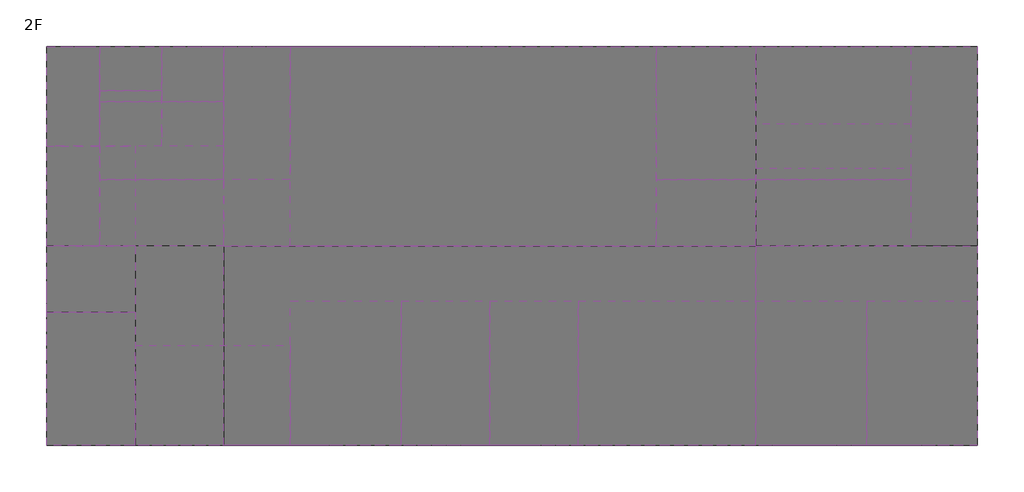
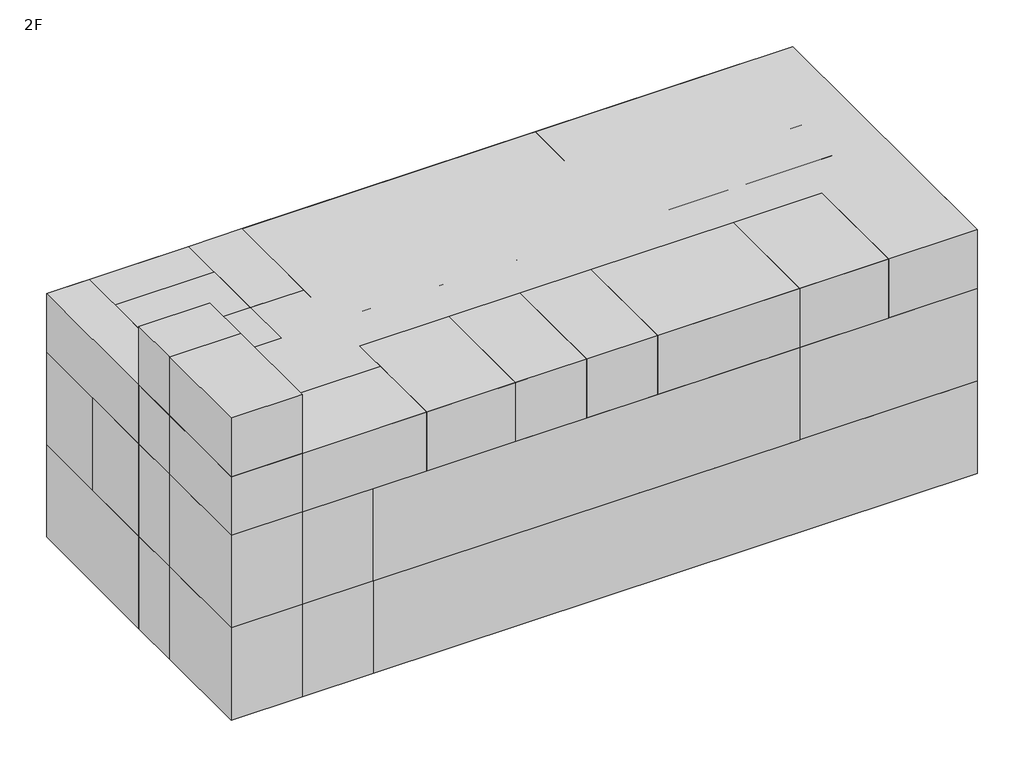
# One storey: 39 proxies.
"""IFC4 building model written with IfcOpenShell, lengths in millimetres."""

import ifcopenshell
import ifcopenshell.guid

model = None  # the IFC model being written
_history = None  # IfcOwnerHistory: only IFC2X3 demands one
_inside = {}  # id of a spatial element -> (the spatial element, [elements in it])
_under = {}  # id of a project, library or spatial element -> (it, [spatial elements below it])
_declared = {}  # id of a project -> (the project, [libraries it declares])
_typed = {}  # id of a type object -> (the type object, [elements of that type])
_made_of = {}  # id of a material, layer set ... -> (it, [elements and type objects made of it])


def new_model(schema):
    """Start an empty IFC model of exactly this schema.

    Asked for "IFC4X3", IfcOpenShell would pick the latest addendum, in which some entities
    have other attributes; the version numbers below select the first issue.
    IFC2X3 requires an IfcOwnerHistory on every rooted entity: one is made here for all.
    """
    global model, _history
    if schema == "IFC4X3":
        model = ifcopenshell.file(schema_version=(4, 3, 0, 0))
    else:
        model = ifcopenshell.file(schema=schema)
    _inside.clear()
    _under.clear()
    _declared.clear()
    _typed.clear()
    _made_of.clear()
    _history = None
    if model.schema == "IFC2X3":
        org = make("IfcOrganization", Name="unknown")
        user = make(
            "IfcPersonAndOrganization",
            ThePerson=make("IfcPerson", FamilyName="unknown"),
            TheOrganization=org,
        )
        app = make(
            "IfcApplication",
            ApplicationDeveloper=org,
            Version="unknown",
            ApplicationFullName="unknown",
            ApplicationIdentifier="unknown",
        )
        _history = make(
            "IfcOwnerHistory",
            OwningUser=user,
            OwningApplication=app,
            ChangeAction="ADDED",
            CreationDate=0,
        )
    return model


def make(cls, **values):
    """One entity of the class cls with the attributes given. An attribute that is None is left unset."""
    return model.create_entity(
        cls, **{name: value for name, value in values.items() if value is not None}
    )


def rooted(cls, **values):
    """An entity with a GlobalId (a new one), such as an element, a storey or a relation."""
    return make(cls, GlobalId=ifcopenshell.guid.new(), OwnerHistory=_history, **values)


def si_unit(unit_type, name, prefix=None):
    """IfcSIUnit, for example si_unit("LENGTHUNIT", "METRE", prefix="MILLI")."""
    return make("IfcSIUnit", UnitType=unit_type, Prefix=prefix, Name=name)


def assignment(units):
    """IfcUnitAssignment: the units of a project."""
    return None if units is None else make("IfcUnitAssignment", Units=units)


def point(xyz):
    """IfcCartesianPoint."""
    return None if xyz is None else make("IfcCartesianPoint", Coordinates=xyz)


def direction(xyz):
    """IfcDirection."""
    return None if xyz is None else make("IfcDirection", DirectionRatios=xyz)


def frame(location, z_axis=None, x_axis=None):
    """IfcAxis2Placement3D, a coordinate frame: its origin and axes. An axis left out is left unset."""
    return make(
        "IfcAxis2Placement3D",
        Location=point(location),
        Axis=direction(z_axis),
        RefDirection=direction(x_axis),
    )


def origin():
    """The frame at (0, 0, 0) with its axes left unset."""
    return frame((0.0, 0.0, 0.0))


def origin_with_axes():
    """The frame at (0, 0, 0) with the z axis (0, 0, 1) and the x axis (1, 0, 0) written out."""
    return frame((0.0, 0.0, 0.0), z_axis=(0.0, 0.0, 1.0), x_axis=(1.0, 0.0, 0.0))


def place(relative_to, where):
    """IfcLocalPlacement: puts the frame where relative to a parent placement (None: the world)."""
    return make(
        "IfcLocalPlacement", PlacementRelTo=relative_to, RelativePlacement=where
    )


def context(
    kind, dimensions, precision=None, world=None, true_north=None, identifier=None
):
    """IfcGeometricRepresentationContext, for example the 3D "Model" context."""
    return make(
        "IfcGeometricRepresentationContext",
        ContextIdentifier=identifier,
        ContextType=kind,
        CoordinateSpaceDimension=dimensions,
        Precision=precision,
        WorldCoordinateSystem=world,
        TrueNorth=true_north,
    )


def project(units=None, contexts=None):
    """IfcProject with its units and contexts."""
    return rooted(
        "IfcProject",
        Name="project",
        RepresentationContexts=contexts,
        UnitsInContext=assignment(units),
    )


def spatial(cls, under=None, at=None, **own):
    """A site, building, storey or space (cls), placed at a placement, below another one or the project."""
    s = rooted(cls, ObjectPlacement=at, **own)
    if under is not None:
        _under.setdefault(under.id(), (under, []))[1].append(s)
    return s


def polyline(points):
    """IfcPolyline through the points."""
    return make("IfcPolyline", Points=[point(p) for p in points])


def outline(outer, holes=None, kind="AREA"):
    """IfcArbitraryClosedProfileDef: a profile drawn as a closed curve; with holes, ...WithVoids."""
    if holes is None:
        return make("IfcArbitraryClosedProfileDef", ProfileType=kind, OuterCurve=outer)
    return make(
        "IfcArbitraryProfileDefWithVoids",
        ProfileType=kind,
        OuterCurve=outer,
        InnerCurves=holes,
    )


def extrude(swept, where, along, depth):
    """IfcExtrudedAreaSolid: the profile swept, set in the frame where, extruded along a direction by depth."""
    return make(
        "IfcExtrudedAreaSolid",
        SweptArea=swept,
        Position=where,
        ExtrudedDirection=direction(along),
        Depth=depth,
    )


def shape(context_of_items, identifier, shape_type, items):
    """IfcShapeRepresentation: the items that make up one representation, for example the "Body"."""
    return make(
        "IfcShapeRepresentation",
        ContextOfItems=context_of_items,
        RepresentationIdentifier=identifier,
        RepresentationType=shape_type,
        Items=items,
    )


def source(mapping_origin, context_of_items, identifier, shape_type, items):
    """IfcRepresentationMap: a shape defined once, which mapped items show again and again."""
    return make(
        "IfcRepresentationMap",
        MappingOrigin=mapping_origin,
        MappedRepresentation=shape(context_of_items, identifier, shape_type, items),
    )


def transform(
    local_origin,
    x_axis=None,
    y_axis=None,
    z_axis=None,
    scale=None,
    scale2=None,
    scale3=None,
    uniform=True,
):
    """IfcCartesianTransformationOperator3D, or its non-uniform kind. x_axis, y_axis, z_axis: its Axis1, 2, 3."""
    if uniform:
        return make(
            "IfcCartesianTransformationOperator3D",
            Axis1=direction(x_axis),
            Axis2=direction(y_axis),
            LocalOrigin=point(local_origin),
            Scale=scale,
            Axis3=direction(z_axis),
        )
    return make(
        "IfcCartesianTransformationOperator3DnonUniform",
        Axis1=direction(x_axis),
        Axis2=direction(y_axis),
        LocalOrigin=point(local_origin),
        Scale=scale,
        Axis3=direction(z_axis),
        Scale2=scale2,
        Scale3=scale3,
    )


def mapped(mapping_source, mapping_target):
    """IfcMappedItem: shows the shape of a source again, moved by a transform."""
    return make(
        "IfcMappedItem", MappingSource=mapping_source, MappingTarget=mapping_target
    )


def made_of(thing, what):
    """Note that an element or type object is made of a material, layer set ...; save() writes the relation."""
    if what is not None:
        _made_of.setdefault(what.id(), (what, []))[1].append(thing)
    return thing


def element(
    cls,
    number,
    at=None,
    inside=None,
    cuts=None,
    type_object=None,
    material=None,
    context=None,
    identifier="Body",
    shape_type=None,
    held_by="IfcProductDefinitionShape",
    body=None,
    shapes=None,
    **own,
):
    """One element of the class cls, such as IfcWall. Its Tag is "e" and its number.

    at: its placement. inside: the storey or other place that contains it. cuts: it is an
    opening in that element (IfcRelVoidsElement). A single representation is given by context,
    identifier, shape_type and body (its items); several are given by shapes. held_by: the class
    of the entity that holds the representations. save() writes the other relations.
    """
    e = rooted(cls, Tag="e%d" % number, ObjectPlacement=at, **own)
    if body is not None:
        shapes = [shape(context, identifier, shape_type, body)]
    if shapes is not None:
        e.Representation = make(held_by, Representations=shapes)
    if inside is not None:
        _inside.setdefault(inside.id(), (inside, []))[1].append(e)
    if cuts is not None:
        rooted(
            "IfcRelVoidsElement", RelatingBuildingElement=cuts, RelatedOpeningElement=e
        )
    if type_object is not None:
        _typed.setdefault(type_object.id(), (type_object, []))[1].append(e)
    return made_of(e, material)


def aggregate(whole, parts):
    """IfcRelAggregates: a whole, such as a stair, and the parts it consists of."""
    return rooted("IfcRelAggregates", RelatingObject=whole, RelatedObjects=parts)


def save(model, path):
    """Write the relations noted so far, then the file.

    IfcRelAggregates (storeys below a building ...), IfcRelContainedInSpatialStructure (elements
    in a storey), IfcRelDefinesByType, IfcRelAssociatesMaterial and IfcRelDeclares: one each for
    every whole, place, type object, material and project.
    """
    for whole, parts in _under.values():
        aggregate(whole, parts)
    for where, things in _inside.values():
        rooted(
            "IfcRelContainedInSpatialStructure",
            RelatedElements=things,
            RelatingStructure=where,
        )
    for kind, things in _typed.values():
        rooted("IfcRelDefinesByType", RelatedObjects=things, RelatingType=kind)
    for what, things in _made_of.values():
        rooted("IfcRelAssociatesMaterial", RelatedObjects=things, RelatingMaterial=what)
    for by, libraries in _declared.values():
        rooted("IfcRelDeclares", RelatingContext=by, RelatedDefinitions=libraries)
    model.write(path)


def generic_models_c89eb543(model_context):
    return source(origin(), model_context, "Body", "SweptSolid", [
        extrude(outline(polyline([(2000.0, 3000.0), (2000.0, -3000.0), (-2000.0, -3000.0), (-2000.0, 3000.0), (2000.0, 3000.0)])), origin_with_axes(), (0.0, 0.0, 1.0), 3500.0),
    ])


def generic_models_50f5a469(model_context):
    return source(origin(), model_context, "Body", "SweptSolid", [
        extrude(outline(polyline([(4500.0, 16000.0), (4500.0, -16000.0), (-4500.0, -16000.0), (-4500.0, 16000.0), (4500.0, 16000.0)])), origin_with_axes(), (0.0, 0.0, 1.0), 5500.0),
    ])


def generic_models_8b5775ea(model_context):
    return source(origin(), model_context, "Body", "SweptSolid", [
        extrude(outline(polyline([(4500.0, 17000.0), (4500.0, -17000.0), (-4500.0, -17000.0), (-4500.0, 17000.0), (4500.0, 17000.0)])), origin_with_axes(), (0.0, 0.0, 1.0), 5500.0),
    ])


def generic_models_2d265e4a(model_context):
    return source(origin(), model_context, "Body", "SweptSolid", [
        extrude(outline(polyline([(4500.0, 5000.0), (4500.0, -5000.0), (-4500.0, -5000.0), (-4500.0, 5000.0), (4500.0, 5000.0)])), origin_with_axes(), (0.0, 0.0, 1.0), 5500.0),
    ])


def generic_models_8934d72c(model_context):
    return source(origin(), model_context, "Body", "SweptSolid", [
        extrude(outline(polyline([(2000.0, 4500.0), (2000.0, -4500.0), (-2000.0, -4500.0), (-2000.0, 4500.0), (2000.0, 4500.0)])), origin_with_axes(), (0.0, 0.0, 1.0), 5500.0),
    ])


def generic_models_626d8198(model_context):
    return source(origin(), model_context, "Body", "SweptSolid", [
        extrude(outline(polyline([(2000.0, 1500.0), (2000.0, -1500.0), (-2000.0, -1500.0), (-2000.0, 1500.0), (2000.0, 1500.0)])), origin_with_axes(), (0.0, 0.0, 1.0), 5500.0),
    ])


def generic_models_cc1dae17(model_context):
    return source(origin(), model_context, "Body", "SweptSolid", [
        extrude(outline(polyline([(2000.0, 3000.0), (2000.0, -3000.0), (-2000.0, -3000.0), (-2000.0, 3000.0), (2000.0, 3000.0)])), origin_with_axes(), (0.0, 0.0, 1.0), 5500.0),
    ])


def generic_models_7ea3b148(model_context):
    return source(origin(), model_context, "Body", "SweptSolid", [
        extrude(outline(polyline([(4500.0, 12000.0), (4500.0, -12000.0), (-4500.0, -12000.0), (-4500.0, 12000.0), (4500.0, 12000.0)])), origin_with_axes(), (0.0, 0.0, 1.0), 5500.0),
    ])


def generic_models_85ff21bb(model_context):
    return source(origin(), model_context, "Body", "SweptSolid", [
        extrude(outline(polyline([(3500.0, 1750.0), (3500.0, -1750.0), (-3500.0, -1750.0), (-3500.0, 1750.0), (3500.0, 1750.0)])), origin_with_axes(), (0.0, 0.0, 1.0), 5500.0),
    ])


def generic_models_570012e4(model_context):
    return source(origin(), model_context, "Body", "SweptSolid", [
        extrude(outline(polyline([(1200.0, 2250.0), (1200.0, -2250.0), (-1200.0, -2250.0), (-1200.0, 2250.0), (1200.0, 2250.0)])), origin_with_axes(), (0.0, 0.0, 1.0), 5500.0),
    ])


def generic_models_971c0b89(model_context):
    return source(origin(), model_context, "Body", "SweptSolid", [
        extrude(outline(polyline([(2000.0, 2250.0), (2000.0, -2250.0), (-2000.0, -2250.0), (-2000.0, 2250.0), (2000.0, 2250.0)])), origin_with_axes(), (0.0, 0.0, 1.0), 5500.0),
    ])


def generic_models_ac48a1a3(model_context):
    return source(origin(), model_context, "Body", "SweptSolid", [
        extrude(outline(polyline([(1400.0, 2250.0), (1400.0, -2250.0), (-1400.0, -2250.0), (-1400.0, 2250.0), (1400.0, 2250.0)])), origin_with_axes(), (0.0, 0.0, 1.0), 5500.0),
    ])


def generic_models_ee32b0c6(model_context):
    return source(origin(), model_context, "Body", "SweptSolid", [
        extrude(outline(polyline([(1400.0, 1000.0), (1400.0, -1000.0), (-1400.0, -1000.0), (-1400.0, 1000.0), (1400.0, 1000.0)])), origin_with_axes(), (0.0, 0.0, 1.0), 5500.0),
    ])


def generic_models_0ee3397c(model_context):
    return source(origin(), model_context, "Body", "SweptSolid", [
        extrude(outline(polyline([(1400.0, 1250.0), (1400.0, -1250.0), (-1400.0, -1250.0), (-1400.0, 1250.0), (1400.0, 1250.0)])), origin_with_axes(), (0.0, 0.0, 1.0), 5500.0),
    ])


def generic_models_8c4134a9(model_context):
    return source(origin(), model_context, "Body", "SweptSolid", [
        extrude(outline(polyline([(3250.0, 2000.0), (3250.0, -2000.0), (-3250.0, -2000.0), (-3250.0, 2000.0), (3250.0, 2000.0)])), origin_with_axes(), (0.0, 0.0, 1.0), 3500.0),
    ])


def generic_models_ccc8c8c2(model_context):
    return source(origin(), model_context, "Body", "SweptSolid", [
        extrude(outline(polyline([(3000.0, 5750.0), (3000.0, -5750.0), (-3000.0, -5750.0), (-3000.0, 5750.0), (3000.0, 5750.0)])), origin_with_axes(), (0.0, 0.0, 1.0), 3500.0),
    ])


def generic_models_70f6ae48(model_context):
    return source(origin(), model_context, "Body", "SweptSolid", [
        extrude(outline(polyline([(3250.0, 4000.0), (3250.0, -4000.0), (-3250.0, -4000.0), (-3250.0, 4000.0), (3250.0, 4000.0)])), origin_with_axes(), (0.0, 0.0, 1.0), 3500.0),
    ])


def generic_models_f0561c1d(model_context):
    return source(origin(), model_context, "Body", "SweptSolid", [
        extrude(outline(polyline([(4500.0, 8250.0), (4500.0, -8250.0), (-4500.0, -8250.0), (-4500.0, 8250.0), (4500.0, 8250.0)])), origin_with_axes(), (0.0, 0.0, 1.0), 3500.0),
    ])


def generic_models_249c6621(model_context):
    return source(origin(), model_context, "Body", "SweptSolid", [
        extrude(outline(polyline([(3250.0, 2500.0), (3250.0, -2500.0), (-3250.0, -2500.0), (-3250.0, 2500.0), (3250.0, 2500.0)])), origin_with_axes(), (0.0, 0.0, 1.0), 3500.0),
    ])


def generic_models_f1f4091a(model_context):
    return source(origin(), model_context, "Body", "SweptSolid", [
        extrude(outline(polyline([(1500.0, 5750.0), (1500.0, -5750.0), (-1500.0, -5750.0), (-1500.0, 5750.0), (1500.0, 5750.0)])), origin_with_axes(), (0.0, 0.0, 1.0), 3500.0),
    ])


def generic_models_10b6925f(model_context):
    return source(origin(), model_context, "Body", "SweptSolid", [
        extrude(outline(polyline([(2250.0, 3500.0), (2250.0, -3500.0), (-2250.0, -3500.0), (-2250.0, 3500.0), (2250.0, 3500.0)])), origin_with_axes(), (0.0, 0.0, 1.0), 3500.0),
    ])


def generic_models_b37916ea(model_context):
    return source(origin(), model_context, "Body", "SweptSolid", [
        extrude(outline(polyline([(1750.0, 2800.0), (1750.0, -2800.0), (-1750.0, -2800.0), (-1750.0, 2800.0), (1750.0, 2800.0)])), origin_with_axes(), (0.0, 0.0, 1.0), 3500.0),
    ])


def generic_models_6c75c912(model_context):
    return source(origin(), model_context, "Body", "SweptSolid", [
        extrude(outline(polyline([(1250.0, 2800.0), (1250.0, -2800.0), (-1250.0, -2800.0), (-1250.0, 2800.0), (1250.0, 2800.0)])), origin_with_axes(), (0.0, 0.0, 1.0), 3500.0),
    ])


def generic_models_a5818909(model_context):
    return source(origin(), model_context, "Body", "SweptSolid", [
        extrude(outline(polyline([(3000.0, 1500.0), (3000.0, -1500.0), (-3000.0, -1500.0), (-3000.0, 1500.0), (3000.0, 1500.0)])), origin_with_axes(), (0.0, 0.0, 1.0), 3500.0),
    ])


def generic_models_f42d0df8(model_context):
    return source(origin(), model_context, "Body", "SweptSolid", [
        extrude(outline(polyline([(1500.0, 2800.0), (1500.0, -2800.0), (-1500.0, -2800.0), (-1500.0, 2800.0), (1500.0, 2800.0)])), origin_with_axes(), (0.0, 0.0, 1.0), 3500.0),
    ])


def generic_models_3f6e5246(model_context):
    return source(origin(), model_context, "Body", "SweptSolid", [
        extrude(outline(polyline([(1200.0, 4500.0), (1200.0, -4500.0), (-1200.0, -4500.0), (-1200.0, 4500.0), (1200.0, 4500.0)])), origin_with_axes(), (0.0, 0.0, 1.0), 3500.0),
    ])


def generic_models_4c644d41(model_context):
    return source(origin(), model_context, "Body", "SweptSolid", [
        extrude(outline(polyline([(2000.0, 1500.0), (2000.0, -1500.0), (-2000.0, -1500.0), (-2000.0, 1500.0), (2000.0, 1500.0)])), origin_with_axes(), (0.0, 0.0, 1.0), 3500.0),
    ])


def generic_models_3d03af35(model_context):
    return source(origin(), model_context, "Body", "SweptSolid", [
        extrude(outline(polyline([(21000.0, 9000.0), (21000.0, -9000.0), (-21000.0, -9000.0), (-21000.0, 9000.0), (21000.0, 9000.0)])), origin_with_axes(), (0.0, 0.0, 1.0), 5500.0),
    ])


def generic_models_bb515c93(model_context):
    return source(origin(), model_context, "Body", "SweptSolid", [
        extrude(outline(polyline([(9000.0, 21000.0), (9000.0, -21000.0), (-9000.0, -21000.0), (-9000.0, 21000.0), (9000.0, 21000.0)])), origin_with_axes(), (0.0, 0.0, 1.0), 3500.0),
    ])


model = new_model("IFC4")

# Units and contexts
model_context = context("Model", 3, world=origin())
ifc_project = project(units=[si_unit("LENGTHUNIT", "METRE", prefix="MILLI")], contexts=[model_context])

# Site, building, storey
site = spatial("IfcSite", under=ifc_project)
building = spatial("IfcBuilding", under=site)
storey = spatial("IfcBuildingStorey", under=building, Name="2F", Elevation=3500.0)

# Proxies
placement = place(None, origin())
generic_models_shape = generic_models_c89eb543(model_context)
element("IfcBuildingElementProxy", 1, Name="Space Planning Box_hec : Space Planning Box_hec", ObjectType="Space Planning Box_hec : Space Planning Box_hec", at=placement, inside=storey, context=model_context, shape_type="MappedRepresentation", body=[
    mapped(generic_models_shape, transform((47459.6521483, 166923.8614395, 14500.0), x_axis=(1.0, 0.0, 0.0), y_axis=(0.0, 1.0, 0.0), z_axis=(0.0, 0.0, 1.0))),
])
element("IfcBuildingElementProxy", 2, Name="Space Planning Box_hec : Space Planning Box_hec", ObjectType="Space Planning Box_hec : Space Planning Box_hec", at=placement, inside=storey, context=model_context, shape_type="MappedRepresentation", body=[
    mapped(generic_models_shape, transform((47459.6521483, 166923.8614395, 18000.0), x_axis=(1.0, 0.0, 0.0), y_axis=(0.0, 1.0, 0.0), z_axis=(0.0, 0.0, 1.0))),
])
generic_models_2_shape = generic_models_50f5a469(model_context)
element("IfcBuildingElementProxy", 3, Name="Space Planning Box_hec : Space Planning Box_hec", ObjectType="Space Planning Box_hec : Space Planning Box_hec", at=placement, inside=storey, context=model_context, shape_type="MappedRepresentation", body=[
    mapped(generic_models_2_shape, transform((61459.6521483, 177423.8614395, 3500.0), x_axis=(0.0, 1.0, 0.0), y_axis=(-1.0, 0.0, 0.0), z_axis=(0.0, 0.0, 1.0))),
])
generic_models_3_shape = generic_models_8b5775ea(model_context)
element("IfcBuildingElementProxy", 4, Name="Space Planning Box_hec : Space Planning Box_hec", ObjectType="Space Planning Box_hec : Space Planning Box_hec", at=placement, inside=storey, context=model_context, shape_type="MappedRepresentation", body=[
    mapped(generic_models_3_shape, transform((70459.6521483, 168423.8614395, 3500.0), x_axis=(0.0, 1.0, 0.0), y_axis=(-1.0, 0.0, 0.0), z_axis=(0.0, 0.0, 1.0))),
])
generic_models_4_shape = generic_models_2d265e4a(model_context)
element("IfcBuildingElementProxy", 5, Name="Space Planning Box_hec : Space Planning Box_hec", ObjectType="Space Planning Box_hec : Space Planning Box_hec", at=placement, inside=storey, context=model_context, shape_type="MappedRepresentation", body=[
    mapped(generic_models_4_shape, transform((82459.6521483, 177423.8614395, 3500.0), x_axis=(0.0, 1.0, 0.0), y_axis=(-1.0, 0.0, 0.0), z_axis=(0.0, 0.0, 1.0))),
])
generic_models_5_shape = generic_models_8934d72c(model_context)
element("IfcBuildingElementProxy", 6, Name="Space Planning Box_hec : Space Planning Box_hec", ObjectType="Space Planning Box_hec : Space Planning Box_hec", at=placement, inside=storey, context=model_context, shape_type="MappedRepresentation", body=[
    mapped(generic_models_5_shape, transform((51459.6521483, 168423.8614395, 3500.0), x_axis=(1.0, 0.0, 0.0), y_axis=(0.0, 1.0, 0.0), z_axis=(0.0, 0.0, 1.0))),
])
generic_models_6_shape = generic_models_626d8198(model_context)
element("IfcBuildingElementProxy", 7, Name="Space Planning Box_hec : Space Planning Box_hec", ObjectType="Space Planning Box_hec : Space Planning Box_hec", at=placement, inside=storey, context=model_context, shape_type="MappedRepresentation", body=[
    mapped(generic_models_6_shape, transform((47459.6521483, 171423.8614395, 3500.0), x_axis=(1.0, 0.0, 0.0), y_axis=(0.0, 1.0, 0.0), z_axis=(0.0, 0.0, 1.0))),
])
element("IfcBuildingElementProxy", 8, Name="Space Planning Box_hec : Space Planning Box_hec", ObjectType="Space Planning Box_hec : Space Planning Box_hec", at=placement, inside=storey, context=model_context, shape_type="MappedRepresentation", body=[
    mapped(generic_models_6_shape, transform((47459.6521483, 171423.8614395, 9000.0), x_axis=(1.0, 0.0, 0.0), y_axis=(0.0, 1.0, 0.0), z_axis=(0.0, 0.0, 1.0))),
])
generic_models_7_shape = generic_models_cc1dae17(model_context)
element("IfcBuildingElementProxy", 9, Name="Space Planning Box_hec : Space Planning Box_hec", ObjectType="Space Planning Box_hec : Space Planning Box_hec", at=placement, inside=storey, context=model_context, shape_type="MappedRepresentation", body=[
    mapped(generic_models_7_shape, transform((47459.6521483, 166923.8614395, 3500.0), x_axis=(1.0, 0.0, 0.0), y_axis=(0.0, 1.0, 0.0), z_axis=(0.0, 0.0, 1.0))),
])
element("IfcBuildingElementProxy", 10, Name="Space Planning Box_hec : Space Planning Box_hec", ObjectType="Space Planning Box_hec : Space Planning Box_hec", at=placement, inside=storey, context=model_context, shape_type="MappedRepresentation", body=[
    mapped(generic_models_7_shape, transform((47459.6521483, 166923.8614395, 9000.0), x_axis=(1.0, 0.0, 0.0), y_axis=(0.0, 1.0, 0.0), z_axis=(0.0, 0.0, 1.0))),
])
generic_models_8_shape = generic_models_7ea3b148(model_context)
element("IfcBuildingElementProxy", 11, Name="Space Planning Box_hec : Space Planning Box_hec", ObjectType="Space Planning Box_hec : Space Planning Box_hec", at=placement, inside=storey, context=model_context, shape_type="MappedRepresentation", body=[
    mapped(generic_models_8_shape, transform((65459.6521483, 177423.8614395, 9000.0), x_axis=(0.0, -1.0, 0.0), y_axis=(1.0, 0.0, 0.0), z_axis=(0.0, 0.0, 1.0))),
])
element("IfcBuildingElementProxy", 12, Name="Space Planning Box_hec : Space Planning Box_hec", ObjectType="Space Planning Box_hec : Space Planning Box_hec", at=placement, inside=storey, context=model_context, shape_type="MappedRepresentation", body=[
    mapped(generic_models_8_shape, transform((65459.6521483, 168423.8614395, 9000.0), x_axis=(0.0, -1.0, 0.0), y_axis=(1.0, 0.0, 0.0), z_axis=(0.0, 0.0, 1.0))),
])
generic_models_9_shape = generic_models_85ff21bb(model_context)
element("IfcBuildingElementProxy", 13, Name="Space Planning Box_hec : Space Planning Box_hec", ObjectType="Space Planning Box_hec : Space Planning Box_hec", at=placement, inside=storey, context=model_context, shape_type="MappedRepresentation", body=[
    mapped(generic_models_9_shape, transform((80959.6521483, 180173.8614395, 9000.0), x_axis=(1.0, 0.0, 0.0), y_axis=(0.0, 1.0, 0.0), z_axis=(0.0, 0.0, 1.0))),
])
element("IfcBuildingElementProxy", 14, Name="Space Planning Box_hec : Space Planning Box_hec", ObjectType="Space Planning Box_hec : Space Planning Box_hec", at=placement, inside=storey, context=model_context, shape_type="MappedRepresentation", body=[
    mapped(generic_models_4_shape, transform((82459.6521483, 168423.8614395, 9000.0), x_axis=(0.0, 1.0, 0.0), y_axis=(-1.0, 0.0, 0.0), z_axis=(0.0, 0.0, 1.0))),
])
element("IfcBuildingElementProxy", 15, Name="Space Planning Box_hec : Space Planning Box_hec", ObjectType="Space Planning Box_hec : Space Planning Box_hec", at=placement, inside=storey, context=model_context, shape_type="MappedRepresentation", body=[
    mapped(generic_models_9_shape, transform((80959.6521483, 174673.8614395, 9000.0), x_axis=(1.0, 0.0, 0.0), y_axis=(0.0, 1.0, 0.0), z_axis=(0.0, 0.0, 1.0))),
])
generic_models_10_shape = generic_models_570012e4(model_context)
element("IfcBuildingElementProxy", 16, Name="Space Planning Box_hec : Space Planning Box_hec", ObjectType="Space Planning Box_hec : Space Planning Box_hec", at=placement, inside=storey, context=model_context, shape_type="MappedRepresentation", body=[
    mapped(generic_models_10_shape, transform((46659.6521483, 179673.8614395, 9000.0), x_axis=(1.0, 0.0, 0.0), y_axis=(0.0, 1.0, 0.0), z_axis=(0.0, 0.0, 1.0))),
])
generic_models_11_shape = generic_models_971c0b89(model_context)
element("IfcBuildingElementProxy", 17, Name="Space Planning Box_hec : Space Planning Box_hec", ObjectType="Space Planning Box_hec : Space Planning Box_hec", at=placement, inside=storey, context=model_context, shape_type="MappedRepresentation", body=[
    mapped(generic_models_11_shape, transform((47459.6521483, 175173.8614395, 9000.0), x_axis=(1.0, 0.0, 0.0), y_axis=(0.0, 1.0, 0.0), z_axis=(0.0, 0.0, 1.0))),
])
generic_models_12_shape = generic_models_ac48a1a3(model_context)
element("IfcBuildingElementProxy", 18, Name="Space Planning Box_hec : Space Planning Box_hec", ObjectType="Space Planning Box_hec : Space Planning Box_hec", at=placement, inside=storey, context=model_context, shape_type="MappedRepresentation", body=[
    mapped(generic_models_12_shape, transform((52059.6521483, 179673.8614395, 9000.0), x_axis=(1.0, 0.0, 0.0), y_axis=(0.0, 1.0, 0.0), z_axis=(0.0, 0.0, 1.0))),
])
generic_models_13_shape = generic_models_ee32b0c6(model_context)
element("IfcBuildingElementProxy", 19, Name="Space Planning Box_hec : Space Planning Box_hec", ObjectType="Space Planning Box_hec : Space Planning Box_hec", at=placement, inside=storey, context=model_context, shape_type="MappedRepresentation", body=[
    mapped(generic_models_13_shape, transform((49259.6521483, 180923.8614395, 9000.0), x_axis=(1.0, 0.0, 0.0), y_axis=(0.0, 1.0, 0.0), z_axis=(0.0, 0.0, 1.0))),
])
generic_models_14_shape = generic_models_0ee3397c(model_context)
element("IfcBuildingElementProxy", 20, Name="Space Planning Box_hec : Space Planning Box_hec", ObjectType="Space Planning Box_hec : Space Planning Box_hec", at=placement, inside=storey, context=model_context, shape_type="MappedRepresentation", body=[
    mapped(generic_models_14_shape, transform((49259.6521483, 178673.8614395, 9000.0), x_axis=(1.0, 0.0, 0.0), y_axis=(0.0, 1.0, 0.0), z_axis=(0.0, 0.0, 1.0))),
])
generic_models_15_shape = generic_models_8c4134a9(model_context)
element("IfcBuildingElementProxy", 21, Name="Space Planning Box_hec : Space Planning Box_hec", ObjectType="Space Planning Box_hec : Space Planning Box_hec", at=placement, inside=storey, context=model_context, shape_type="MappedRepresentation", body=[
    mapped(generic_models_15_shape, transform((63459.6521483, 167173.8614395, 14500.0), x_axis=(0.0, 1.0, 0.0), y_axis=(-1.0, 0.0, 0.0), z_axis=(0.0, 0.0, 1.0))),
])
element("IfcBuildingElementProxy", 22, Name="Space Planning Box_hec : Space Planning Box_hec", ObjectType="Space Planning Box_hec : Space Planning Box_hec", at=placement, inside=storey, context=model_context, shape_type="MappedRepresentation", body=[
    mapped(generic_models_15_shape, transform((67459.6521483, 167173.8614395, 14500.0), x_axis=(0.0, 1.0, 0.0), y_axis=(-1.0, 0.0, 0.0), z_axis=(0.0, 0.0, 1.0))),
])
generic_models_16_shape = generic_models_ccc8c8c2(model_context)
element("IfcBuildingElementProxy", 23, Name="Space Planning Box_hec : Space Planning Box_hec", ObjectType="Space Planning Box_hec : Space Planning Box_hec", at=placement, inside=storey, context=model_context, shape_type="MappedRepresentation", body=[
    mapped(generic_models_16_shape, transform((78709.6521483, 178923.8614395, 14500.0), x_axis=(0.0, -1.0, 0.0), y_axis=(1.0, 0.0, 0.0), z_axis=(0.0, 0.0, 1.0))),
])
generic_models_17_shape = generic_models_70f6ae48(model_context)
element("IfcBuildingElementProxy", 24, Name="Space Planning Box_hec : Space Planning Box_hec", ObjectType="Space Planning Box_hec : Space Planning Box_hec", at=placement, inside=storey, context=model_context, shape_type="MappedRepresentation", body=[
    mapped(generic_models_17_shape, transform((73459.6521483, 167173.8614395, 14500.0), x_axis=(0.0, -1.0, 0.0), y_axis=(1.0, 0.0, 0.0), z_axis=(0.0, 0.0, 1.0))),
])
generic_models_18_shape = generic_models_f0561c1d(model_context)
element("IfcBuildingElementProxy", 25, Name="Space Planning Box_hec : Space Planning Box_hec", ObjectType="Space Planning Box_hec : Space Planning Box_hec", at=placement, inside=storey, context=model_context, shape_type="MappedRepresentation", body=[
    mapped(generic_models_18_shape, transform((64709.6521483, 177423.8614395, 14500.0), x_axis=(0.0, -1.0, 0.0), y_axis=(1.0, 0.0, 0.0), z_axis=(0.0, 0.0, 1.0))),
])
generic_models_19_shape = generic_models_249c6621(model_context)
element("IfcBuildingElementProxy", 26, Name="Space Planning Box_hec : Space Planning Box_hec", ObjectType="Space Planning Box_hec : Space Planning Box_hec", at=placement, inside=storey, context=model_context, shape_type="MappedRepresentation", body=[
    mapped(generic_models_19_shape, transform((79959.6521483, 167173.8614395, 14500.0), x_axis=(0.0, -1.0, 0.0), y_axis=(1.0, 0.0, 0.0), z_axis=(0.0, 0.0, 1.0))),
])
element("IfcBuildingElementProxy", 27, Name="Space Planning Box_hec : Space Planning Box_hec", ObjectType="Space Planning Box_hec : Space Planning Box_hec", at=placement, inside=storey, context=model_context, shape_type="MappedRepresentation", body=[
    mapped(generic_models_19_shape, transform((58959.6521483, 167173.8614395, 14500.0), x_axis=(0.0, 1.0, 0.0), y_axis=(-1.0, 0.0, 0.0), z_axis=(0.0, 0.0, 1.0))),
])
element("IfcBuildingElementProxy", 28, Name="Space Planning Box_hec : Space Planning Box_hec", ObjectType="Space Planning Box_hec : Space Planning Box_hec", at=placement, inside=storey, context=model_context, shape_type="MappedRepresentation", body=[
    mapped(generic_models_19_shape, transform((84959.6521483, 167173.8614395, 14500.0), x_axis=(0.0, 1.0, 0.0), y_axis=(-1.0, 0.0, 0.0), z_axis=(0.0, 0.0, 1.0))),
])
generic_models_20_shape = generic_models_f1f4091a(model_context)
element("IfcBuildingElementProxy", 29, Name="Space Planning Box_hec : Space Planning Box_hec", ObjectType="Space Planning Box_hec : Space Planning Box_hec", at=placement, inside=storey, context=model_context, shape_type="MappedRepresentation", body=[
    mapped(generic_models_20_shape, transform((78709.6521483, 174423.8614395, 14500.0), x_axis=(0.0, 1.0, 0.0), y_axis=(-1.0, 0.0, 0.0), z_axis=(0.0, 0.0, 1.0))),
])
generic_models_21_shape = generic_models_10b6925f(model_context)
element("IfcBuildingElementProxy", 30, Name="Space Planning Box_hec : Space Planning Box_hec", ObjectType="Space Planning Box_hec : Space Planning Box_hec", at=placement, inside=storey, context=model_context, shape_type="MappedRepresentation", body=[
    mapped(generic_models_21_shape, transform((52959.6521483, 166173.8614395, 14500.0), x_axis=(0.0, -1.0, 0.0), y_axis=(1.0, 0.0, 0.0), z_axis=(0.0, 0.0, 1.0))),
])
generic_models_22_shape = generic_models_b37916ea(model_context)
element("IfcBuildingElementProxy", 31, Name="Space Planning Box_hec : Space Planning Box_hec", ObjectType="Space Planning Box_hec : Space Planning Box_hec", at=placement, inside=storey, context=model_context, shape_type="MappedRepresentation", body=[
    mapped(generic_models_22_shape, transform((50659.6521483, 177673.8614395, 14500.0), x_axis=(0.0, -1.0, 0.0), y_axis=(1.0, 0.0, 0.0), z_axis=(0.0, 0.0, 1.0))),
])
generic_models_23_shape = generic_models_6c75c912(model_context)
element("IfcBuildingElementProxy", 32, Name="Space Planning Box_hec : Space Planning Box_hec", ObjectType="Space Planning Box_hec : Space Planning Box_hec", at=placement, inside=storey, context=model_context, shape_type="MappedRepresentation", body=[
    mapped(generic_models_23_shape, transform((50659.6521483, 180673.8614395, 14500.0), x_axis=(0.0, -1.0, 0.0), y_axis=(1.0, 0.0, 0.0), z_axis=(0.0, 0.0, 1.0))),
])
generic_models_24_shape = generic_models_a5818909(model_context)
element("IfcBuildingElementProxy", 33, Name="Space Planning Box_hec : Space Planning Box_hec", ObjectType="Space Planning Box_hec : Space Planning Box_hec", at=placement, inside=storey, context=model_context, shape_type="MappedRepresentation", body=[
    mapped(generic_models_24_shape, transform((54959.6521483, 178923.8614395, 14500.0), x_axis=(0.0, -1.0, 0.0), y_axis=(1.0, 0.0, 0.0), z_axis=(0.0, 0.0, 1.0))),
])
generic_models_25_shape = generic_models_f42d0df8(model_context)
element("IfcBuildingElementProxy", 34, Name="Space Planning Box_hec : Space Planning Box_hec", ObjectType="Space Planning Box_hec : Space Planning Box_hec", at=placement, inside=storey, context=model_context, shape_type="MappedRepresentation", body=[
    mapped(generic_models_25_shape, transform((50659.6521483, 174423.8614395, 14500.0), x_axis=(0.0, -1.0, 0.0), y_axis=(1.0, 0.0, 0.0), z_axis=(0.0, 0.0, 1.0))),
])
generic_models_26_shape = generic_models_3f6e5246(model_context)
element("IfcBuildingElementProxy", 35, Name="Space Planning Box_hec : Space Planning Box_hec", ObjectType="Space Planning Box_hec : Space Planning Box_hec", at=placement, inside=storey, context=model_context, shape_type="MappedRepresentation", body=[
    mapped(generic_models_26_shape, transform((46659.6521483, 177423.8614395, 14500.0), x_axis=(1.0, 0.0, 0.0), y_axis=(0.0, 1.0, 0.0), z_axis=(0.0, 0.0, 1.0))),
])
generic_models_27_shape = generic_models_4c644d41(model_context)
element("IfcBuildingElementProxy", 36, Name="Space Planning Box_hec : Space Planning Box_hec", ObjectType="Space Planning Box_hec : Space Planning Box_hec", at=placement, inside=storey, context=model_context, shape_type="MappedRepresentation", body=[
    mapped(generic_models_27_shape, transform((47459.6521483, 171423.8614395, 14500.0), x_axis=(1.0, 0.0, 0.0), y_axis=(0.0, 1.0, 0.0), z_axis=(0.0, 0.0, 1.0))),
])
element("IfcBuildingElementProxy", 37, Name="Space Planning Box_hec : Space Planning Box_hec", ObjectType="Space Planning Box_hec : Space Planning Box_hec", at=placement, inside=storey, context=model_context, shape_type="MappedRepresentation", body=[
    mapped(generic_models_27_shape, transform((47459.6521483, 171423.8614395, 18000.0), x_axis=(1.0, 0.0, 0.0), y_axis=(0.0, 1.0, 0.0), z_axis=(0.0, 0.0, 1.0))),
])
generic_models_28_shape = generic_models_3d03af35(model_context)
element("IfcBuildingElementProxy", 38, Name="Space Planning Box_hec : Space Planning Box_hec", ObjectType="Space Planning Box_hec : Space Planning Box_hec", at=placement, inside=storey, context=model_context, shape_type="MappedRepresentation", body=[
    mapped(generic_models_28_shape, transform((66459.6521483, 172923.8614395, 9000.0), x_axis=(1.0, 0.0, 0.0), y_axis=(0.0, 1.0, 0.0), z_axis=(0.0, 0.0, 1.0))),
])
generic_models_29_shape = generic_models_bb515c93(model_context)
element("IfcBuildingElementProxy", 39, Name="Space Planning Box_hec : Space Planning Box_hec", ObjectType="Space Planning Box_hec : Space Planning Box_hec", at=placement, inside=storey, context=model_context, shape_type="MappedRepresentation", body=[
    mapped(generic_models_29_shape, transform((66459.6521483, 172923.8614395, 14500.0), x_axis=(0.0, -1.0, 0.0), y_axis=(1.0, 0.0, 0.0), z_axis=(0.0, 0.0, 1.0))),
])

save(model, "model.ifc")

# Revit data of these elements
# Project information
#   Building Name = "MAIN GATE SECURITY BUILDING"
#   Project Status = "Project Status"
#   Client Name = "현대엔지니어링"
#   Project Address = "서울시 종로구 율곡로 75(계동)"
#   Project Name = "Therma Visayas Energy Project"
#   Project Number = "-"
# Grids (mm)
#   "1": line (45459.652, 190234.526) -> (45459.652, 152139.384)
#   "2": line (53459.652, 190234.526) -> (53459.652, 152139.384)
#   "3": line (61459.652, 190234.526) -> (61459.652, 152139.384)
#   "4": line (69459.652, 190234.526) -> (69459.652, 152139.384)
#   "5": line (77459.652, 190234.526) -> (77459.652, 152139.384)
#   "6": line (87459.652, 190234.526) -> (87459.652, 152139.384)
#   "C": line (39389.066, 181923.861) -> (102402.798, 181923.861)
#   "B": line (39389.066, 172923.861) -> (102402.798, 172923.861)
#   "A": line (39389.066, 163923.861) -> (102402.798, 163923.861)
# Type "Space Planning Box_hec : Space Planning Box_hec"
#   Type Comments = "..."
#   Room Name [instance default] = "?"
#   Interior Finish [instance default] = ""
#   Exterior Finish [instance default] = ""
#   Department [instance default] = ""
#   Assembly Code = "..."
#   ceiling height [instance default] = 0
#   Width [instance default] = 1524 mm
#   Program Area [instance default] = 0.00 m²
#   Length [instance default] = 1524 mm
#   Height [instance default] = 1524 mm
#   Area [instance default] = 2.32258 m²
#   Fill Color [instance default] = Cyan
#   Default Elevation = 0
# Element 1 (IfcBuildingElementProxy, "Space Planning Box_hec : Space Planning Box_hec")
#   Room Name = "Staircase"
#   Interior Finish = "IW5..N/A..N/A,,N/A..N/A,,FL2..N/A,,CL1..N/A"
#   Exterior Finish = "N/A..N/A,,EW2..N/A..N/A"
#   Department = "PATHV1"
#   ceiling height = 0
#   Width = 4000 mm
#   Program Area = 24.00 m²
#   Length = 6000 mm
#   Height = 3500 mm
#   Area = 24.00 m²
#   Fill Color = Green
#   Phase Created = New Construction
#   Materials on its faces: "Green"
# Element 2 (IfcBuildingElementProxy, "Space Planning Box_hec : Space Planning Box_hec")
#   Room Name = "Staircase"
#   Interior Finish = "IW5..N/A..N/A,,WK3..N/A,,FL2..N/A,,N/A..N/A"
#   Exterior Finish = "RF1..N/A,,EW2..EW1..N/A"
#   Department = "PATHV1"
#   ceiling height = 0
#   Width = 4000 mm
#   Program Area = 0.00 m²
#   Length = 6000 mm
#   Height = 3500 mm
#   Area = 24.00 m²
#   Fill Color = Green
#   Phase Created = New Construction
#   Materials on its faces: "Green"
# Element 3 (IfcBuildingElementProxy, "Space Planning Box_hec : Space Planning Box_hec")
#   Room Name = "Electrical Room-1"
#   Interior Finish = "IW5..N/A..N/A,,WK1..N/A,,FL1..N/A,,CL1..N/A"
#   Exterior Finish = "N/A..N/A,,EW1..EW2..N/A"
#   Department = "CI"
#   ceiling height = 0
#   Width = 9000 mm
#   Program Area = 306.00 m²
#   Length = 32000 mm
#   Height = 5500 mm
#   Area = 288.00 m²
#   Fill Color = Yellow
#   Phase Created = New Construction
#   Materials on its faces: "Yellow"
# Element 4 (IfcBuildingElementProxy, "Space Planning Box_hec : Space Planning Box_hec")
#   Room Name = "Electrical Room-2"
#   Interior Finish = "IW5..N/A..N/A,,WK1..N/A,,FL1..N/A,,CL1..N/A"
#   Exterior Finish = "N/A..N/A,,EW1..EW2..N/A"
#   Department = "EL"
#   ceiling height = 0
#   Width = 9000 mm
#   Program Area = 288.00 m²
#   Length = 34000 mm
#   Height = 5500 mm
#   Area = 306.00 m²
#   Fill Color = Orange
#   Phase Created = New Construction
#   Materials on its faces: "Orange"
# Element 5 (IfcBuildingElementProxy, "Space Planning Box_hec : Space Planning Box_hec")
#   Room Name = "Electrical Room (GIS)"
#   Interior Finish = "IW5..N/A..N/A,,WK1..N/A,,FL1..N/A,,CL1..N/A"
#   Exterior Finish = "N/A..N/A,,EW1..EW2..N/A"
#   Department = "AR"
#   ceiling height = 0
#   Width = 9000 mm
#   Program Area = 90.00 m²
#   Length = 10000 mm
#   Height = 5500 mm
#   Area = 90.00 m²
#   Fill Color = Cyan
#   Phase Created = New Construction
#   Materials on its faces: "Cyan"
# Element 6 (IfcBuildingElementProxy, "Space Planning Box_hec : Space Planning Box_hec")
#   Room Name = "Lobby"
#   Interior Finish = "IW5..N/A..N/A,,WK3..N/A,,FL2..N/A,,CL3..N/A"
#   Exterior Finish = "N/A..N/A,,EW2..N/A..N/A"
#   Department = "AR"
#   ceiling height = 0
#   Width = 4000 mm
#   Program Area = 36.00 m²
#   Length = 9000 mm
#   Height = 5500 mm
#   Area = 36.00 m²
#   Fill Color = Cyan
#   Phase Created = New Construction
#   Materials on its faces: "Cyan"
# Element 7 (IfcBuildingElementProxy, "Space Planning Box_hec : Space Planning Box_hec")
#   Room Name = "Elevator"
#   Interior Finish = "N/A..N/A..N/A,,N/A..N/A,,N/A..N/A,,N/A..N/A"
#   Exterior Finish = "N/A..N/A,,EW2..N/A..N/A"
#   Department = "PATHV2"
#   ceiling height = 0
#   Width = 4000 mm
#   Program Area = 12.00 m²
#   Length = 3000 mm
#   Height = 5500 mm
#   Area = 12.00 m²
#   Fill Color = Blue
#   Phase Created = New Construction
#   Materials on its faces: "Blue"
# Element 8 (IfcBuildingElementProxy, "Space Planning Box_hec : Space Planning Box_hec")
#   Room Name = "Elevator"
#   Interior Finish = "N/A..N/A..N/A,,N/A..N/A,,N/A..N/A,,N/A..N/A"
#   Exterior Finish = "N/A..N/A,,EW2..N/A..N/A"
#   Department = "PATHV2"
#   ceiling height = 2700
#   Width = 4000 mm
#   Program Area = 12.00 m²
#   Length = 3000 mm
#   Height = 5500 mm
#   Area = 12.00 m²
#   Fill Color = Blue
#   Phase Created = New Construction
#   Materials on its faces: "Blue"
# Element 9 (IfcBuildingElementProxy, "Space Planning Box_hec : Space Planning Box_hec")
#   Room Name = "Staircase"
#   Interior Finish = "IW5..N/A..N/A,,WK3..N/A,,FL2..N/A,,CL1..N/A"
#   Exterior Finish = "N/A..N/A,,EW2..N/A..N/A"
#   Department = "PATHV1"
#   ceiling height = 0
#   Width = 4000 mm
#   Program Area = 24.00 m²
#   Length = 6000 mm
#   Height = 5500 mm
#   Area = 24.00 m²
#   Fill Color = Green
#   Phase Created = New Construction
#   Materials on its faces: "Green"
# Element 10 (IfcBuildingElementProxy, "Space Planning Box_hec : Space Planning Box_hec")
#   Room Name = "Staircase"
#   Interior Finish = "IW5..N/A..N/A,,WK3..N/A,,FL2..N/A,,CL1..N/A"
#   Exterior Finish = "N/A..N/A,,EW2..N/A..N/A"
#   Department = "PATHV1"
#   ceiling height = 2700
#   Width = 4000 mm
#   Program Area = 24.00 m²
#   Length = 6000 mm
#   Height = 5500 mm
#   Area = 24.00 m²
#   Fill Color = Green
#   Phase Created = New Construction
#   Materials on its faces: "Green"
# Element 11 (IfcBuildingElementProxy, "Space Planning Box_hec : Space Planning Box_hec")
#   Room Name = "Central Control Room"
#   Interior Finish = "IW5..N/A..N/A,,N/A..N/A,,FL5..N/A,,CL3..N/A"
#   Exterior Finish = "N/A..N/A,,EW1..N/A..N/A"
#   Department = "CI"
#   ceiling height = 3400
#   Width = 9000 mm
#   Program Area = 216.00 m²
#   Length = 24000 mm
#   Height = 5500 mm
#   Area = 216.00 m²
#   Fill Color = Yellow
#   Phase Created = New Construction
#   Materials on its faces: "Yellow"
# Element 12 (IfcBuildingElementProxy, "Space Planning Box_hec : Space Planning Box_hec")
#   Room Name = "Electronic Room"
#   Interior Finish = "IW5..N/A..N/A,,N/A..N/A,,FL5..N/A,,CL3..N/A"
#   Exterior Finish = "N/A..N/A,,EW1..N/A..N/A"
#   Department = "CI"
#   ceiling height = 3000
#   Width = 9000 mm
#   Program Area = 216.00 m²
#   Length = 24000 mm
#   Height = 5500 mm
#   Area = 216.00 m²
#   Fill Color = Yellow
#   Phase Created = New Construction
#   Materials on its faces: "Yellow"
# Element 13 (IfcBuildingElementProxy, "Space Planning Box_hec : Space Planning Box_hec")
#   Room Name = "Computer Room"
#   Interior Finish = "IW5..N/A..N/A,,N/A..N/A,,FL5..N/A,,CL3..N/A"
#   Exterior Finish = "N/A..N/A,,EW2..N/A..N/A"
#   Department = "AR"
#   ceiling height = 2700
#   Width = 7000 mm
#   Program Area = 24.50 m²
#   Length = 3500 mm
#   Height = 5500 mm
#   Area = 24.50 m²
#   Fill Color = Cyan
#   Phase Created = New Construction
#   Materials on its faces: "Cyan"
# Element 14 (IfcBuildingElementProxy, "Space Planning Box_hec : Space Planning Box_hec")
#   Room Name = "Electrical Room -3"
#   Interior Finish = "IW5..N/A..N/A,,N/A..N/A,,FL5,,CL3..N/A"
#   Exterior Finish = "N/A..N/A,,EW2..N/A..N/A"
#   Department = "EL"
#   ceiling height = 0
#   Width = 9000 mm
#   Program Area = 90.00 m²
#   Length = 10000 mm
#   Height = 5500 mm
#   Area = 90.00 m²
#   Fill Color = Orange
#   Phase Created = New Construction
#   Materials on its faces: "Orange"
# Element 15 (IfcBuildingElementProxy, "Space Planning Box_hec : Space Planning Box_hec")
#   Room Name = "Communication Room"
#   Interior Finish = "IW5..N/A..N/A,,N/A..N/A,,FL5..N/A,,CL3..N/A"
#   Exterior Finish = "N/A..N/A,,N/A..N/A..N/A"
#   Department = "CI"
#   ceiling height = 2700
#   Width = 7000 mm
#   Program Area = 24.50 m²
#   Length = 3500 mm
#   Height = 5500 mm
#   Area = 24.50 m²
#   Fill Color = Yellow
#   Phase Created = New Construction
#   Materials on its faces: "Yellow"
# Element 16 (IfcBuildingElementProxy, "Space Planning Box_hec : Space Planning Box_hec")
#   Room Name = "Duct Shaft"
#   Interior Finish = "N/A..N/A..N/A,,N/A..N/A,,N/A..N/A,,N/A..N/A"
#   Exterior Finish = "N/A..N/A,,EW2..N/A..N/A"
#   Department = "PATHV3"
#   ceiling height = 2700
#   Width = 2400 mm
#   Program Area = 10.80 m²
#   Length = 4500 mm
#   Height = 5500 mm
#   Area = 10.80 m²
#   Fill Color = Lavender
#   Phase Created = New Construction
#   Materials on its faces: "Lavender"
# Element 17 (IfcBuildingElementProxy, "Space Planning Box_hec : Space Planning Box_hec")
#   Room Name = "Toilet (M)"
#   Interior Finish = "IW3..N/A..N/A,,N/A..N/A,,FL3..N/A,,CL4..N/A"
#   Exterior Finish = "N/A..N/A,,EW2..N/A..N/A"
#   Department = "AR"
#   ceiling height = 2700
#   Width = 4000 mm
#   Program Area = 18.00 m²
#   Length = 4500 mm
#   Height = 5500 mm
#   Area = 18.00 m²
#   Fill Color = Cyan
#   Phase Created = New Construction
#   Materials on its faces: "Cyan"
# Element 18 (IfcBuildingElementProxy, "Space Planning Box_hec : Space Planning Box_hec")
#   Room Name = "Toilet"
#   Interior Finish = "IW3..N/A..N/A,,N/A..N/A,,FL3..N/A,,CL4..N/A"
#   Exterior Finish = "N/A..N/A,,EW2..N/A..N/A"
#   Department = "AR"
#   ceiling height = 2700
#   Width = 2800 mm
#   Program Area = 12.60 m²
#   Length = 4500 mm
#   Height = 5500 mm
#   Area = 12.60 m²
#   Fill Color = Cyan
#   Phase Created = New Construction
#   Materials on its faces: "Cyan"
# Element 19 (IfcBuildingElementProxy, "Space Planning Box_hec : Space Planning Box_hec")
#   Room Name = "Shower"
#   Interior Finish = "IW3..N/A..N/A,,N/A..N/A,,FL3..N/A,,CL4..N/A"
#   Exterior Finish = "N/A..N/A,,EW2..N/A..N/A"
#   Department = "AR"
#   ceiling height = 2700
#   Width = 2800 mm
#   Program Area = 5.60 m²
#   Length = 2000 mm
#   Height = 5500 mm
#   Area = 5.60 m²
#   Fill Color = Cyan
#   Phase Created = New Construction
#   Materials on its faces: "Cyan"
# Element 20 (IfcBuildingElementProxy, "Space Planning Box_hec : Space Planning Box_hec")
#   Room Name = "Locker(F)"
#   Interior Finish = "IW5..N/A..N/A,,WK3..N/A,,FL2..N/A,,CL3..N/A"
#   Exterior Finish = "N/A..N/A,,N/A..N/A..N/A"
#   Department = "AR"
#   ceiling height = 2700
#   Width = 2800 mm
#   Program Area = 7.00 m²
#   Length = 2500 mm
#   Height = 5500 mm
#   Area = 7.00 m²
#   Fill Color = Cyan
#   Phase Created = New Construction
#   Materials on its faces: "Cyan"
# Element 21 (IfcBuildingElementProxy, "Space Planning Box_hec : Space Planning Box_hec")
#   Room Name = "Manager Office-1"
#   Interior Finish = "IW5..N/A..N/A,,WK3..N/A,,FL2..N/A,,CL3..N/A"
#   Exterior Finish = "RF1..N/A,,EW1..N/A..N/A"
#   Department = "AR"
#   ceiling height = 2700
#   Width = 6500 mm
#   Program Area = 26.00 m²
#   Length = 4000 mm
#   Height = 3500 mm
#   Area = 26.00 m²
#   Fill Color = Cyan
#   Phase Created = New Construction
#   Materials on its faces: "Cyan"
# Element 22 (IfcBuildingElementProxy, "Space Planning Box_hec : Space Planning Box_hec")
#   Room Name = "Manager Office-2"
#   Interior Finish = "IW5..N/A..N/A,,WK3..N/A,,FL2..N/A,,CL3..N/A"
#   Exterior Finish = "RF1..N/A,,EW1..N/A..N/A"
#   Department = "AR"
#   ceiling height = 2700
#   Width = 6500 mm
#   Program Area = 26.00 m²
#   Length = 4000 mm
#   Height = 3500 mm
#   Area = 26.00 m²
#   Fill Color = Cyan
#   Phase Created = New Construction
#   Materials on its faces: "Cyan"
# Element 23 (IfcBuildingElementProxy, "Space Planning Box_hec : Space Planning Box_hec")
#   Room Name = "Meeting Room-1"
#   Interior Finish = "IW5..N/A..N/A,,WK3..N/A,,FL2..N/A,,CL3..N/A"
#   Exterior Finish = "RF1..N/A,,EW1..EW2..N/A"
#   Department = "AR"
#   ceiling height = 2700
#   Width = 6000 mm
#   Program Area = 69.00 m²
#   Length = 11500 mm
#   Height = 3500 mm
#   Area = 69.00 m²
#   Fill Color = Cyan
#   Phase Created = New Construction
#   Materials on its faces: "Cyan"
# Element 24 (IfcBuildingElementProxy, "Space Planning Box_hec : Space Planning Box_hec")
#   Room Name = "Meeting Room-2"
#   Interior Finish = "IW5..N/A..N/A,,WK3..N/A,,FL2..N/A,,CL3..N/A"
#   Exterior Finish = "RF1..N/A,,EW1..N/A..N/A"
#   Department = "AR"
#   ceiling height = 2700
#   Width = 6500 mm
#   Program Area = 52.00 m²
#   Length = 8000 mm
#   Height = 3500 mm
#   Area = 52.00 m²
#   Fill Color = Cyan
#   Phase Created = New Construction
#   Materials on its faces: "Cyan"
# Element 25 (IfcBuildingElementProxy, "Space Planning Box_hec : Space Planning Box_hec")
#   Room Name = "Open Office"
#   Interior Finish = "IW5..N/A..N/A,,WK3..N/A,,FL2..N/A,,CL3..N/A"
#   Exterior Finish = "RF1..N/A,,EW1..N/A..N/A"
#   Department = "HV"
#   ceiling height = 0
#   Width = 9000 mm
#   Program Area = 148.50 m²
#   Length = 16500 mm
#   Height = 3500 mm
#   Area = 148.50 m²
#   Fill Color = Lime
#   Phase Created = New Construction
#   Materials on its faces: "Lime"
# Element 26 (IfcBuildingElementProxy, "Space Planning Box_hec : Space Planning Box_hec")
#   Room Name = "Office-1"
#   Interior Finish = "IW5..N/A..N/A,,WK3..N/A,,FL2..N/A,,CL3..N/A"
#   Exterior Finish = "RF1..N/A,,EW2..N/A..N/A"
#   Department = "AR"
#   ceiling height = 0
#   Width = 6500 mm
#   Program Area = 32.50 m²
#   Length = 5000 mm
#   Height = 3500 mm
#   Area = 32.50 m²
#   Fill Color = Cyan
#   Phase Created = New Construction
#   Materials on its faces: "Cyan"
# Element 27 (IfcBuildingElementProxy, "Space Planning Box_hec : Space Planning Box_hec")
#   Room Name = "Storage"
#   Interior Finish = "IW5..N/A..N/A,,WK3..N/A,,FL2..N/A,,CL3..N/A"
#   Exterior Finish = "RF1..N/A,,EW1..N/A..N/A"
#   Department = "AR"
#   ceiling height = 0
#   Width = 6500 mm
#   Program Area = 32.50 m²
#   Length = 5000 mm
#   Height = 3500 mm
#   Area = 32.50 m²
#   Fill Color = Cyan
#   Phase Created = New Construction
#   Materials on its faces: "Cyan"
# Element 28 (IfcBuildingElementProxy, "Space Planning Box_hec : Space Planning Box_hec")
#   Room Name = "Fire Gas Room"
#   Interior Finish = "IW5..N/A..N/A,,WK1..N/A,,FL1..N/A,,N/A..N/A"
#   Exterior Finish = "RF1..N/A,,EW2..N/A..N/A"
#   Department = "FF"
#   ceiling height = 0
#   Width = 6500 mm
#   Program Area = 32.50 m²
#   Length = 5000 mm
#   Height = 3500 mm
#   Area = 32.50 m²
#   Fill Color = Red
#   Phase Created = New Construction
#   Materials on its faces: "Red"
# Element 29 (IfcBuildingElementProxy, "Space Planning Box_hec : Space Planning Box_hec")
#   Room Name = "Document Room"
#   Interior Finish = "IW5..N/A..N/A,,WK3..N/A,,FL2..N/A,,CL3..N/A"
#   Exterior Finish = "RF1..N/A,,N/A..N/A..N/A"
#   Department = "AR"
#   ceiling height = 0
#   Width = 3000 mm
#   Program Area = 34.50 m²
#   Length = 11500 mm
#   Height = 3500 mm
#   Area = 34.50 m²
#   Fill Color = Cyan
#   Phase Created = New Construction
#   Materials on its faces: "Cyan"
# Element 30 (IfcBuildingElementProxy, "Space Planning Box_hec : Space Planning Box_hec")
#   Room Name = "Break Room"
#   Interior Finish = "IW5..N/A..N/A,,WK3..N/A,,FL2..N/A,,CL3..N/A"
#   Exterior Finish = "RF1..N/A,,EW2..N/A..N/A"
#   Department = "AR"
#   ceiling height = 0
#   Width = 4500 mm
#   Program Area = 31.50 m²
#   Length = 7000 mm
#   Height = 3500 mm
#   Area = 31.50 m²
#   Fill Color = Cyan
#   Phase Created = New Construction
#   Materials on its faces: "Cyan"
# Element 31 (IfcBuildingElementProxy, "Space Planning Box_hec : Space Planning Box_hec")
#   Room Name = "Toilet"
#   Interior Finish = "IW3..N/A..N/A,,N/A..N/A,,FL3..N/A,,CL4..N/A"
#   Exterior Finish = "RF1..N/A,,N/A..N/A..N/A"
#   Department = "AR"
#   ceiling height = 2700
#   Width = 3500 mm
#   Program Area = 19.60 m²
#   Length = 5600 mm
#   Height = 3500 mm
#   Area = 19.60 m²
#   Fill Color = Cyan
#   Phase Created = New Construction
#   Materials on its faces: "Cyan"
# Element 32 (IfcBuildingElementProxy, "Space Planning Box_hec : Space Planning Box_hec")
#   Room Name = "Shower"
#   Interior Finish = "IW3..N/A..N/A,,N/A..N/A,,FL3..N/A,,CL4..N/A"
#   Exterior Finish = "RF1..N/A,,EW2..N/A..N/A"
#   Department = "AR"
#   ceiling height = 2700
#   Width = 2500 mm
#   Program Area = 14.00 m²
#   Length = 5600 mm
#   Height = 3500 mm
#   Area = 14.00 m²
#   Fill Color = Cyan
#   Phase Created = New Construction
#   Materials on its faces: "Cyan"
# Element 33 (IfcBuildingElementProxy, "Space Planning Box_hec : Space Planning Box_hec")
#   Room Name = "Locker(M)"
#   Interior Finish = "IW5..N/A..N/A,,WK3..N/A,,FL2..N/A,,CL3..N/A"
#   Exterior Finish = "RF1..N/A,,EW1..N/A..N/A"
#   Department = "AR"
#   ceiling height = 2700
#   Width = 6000 mm
#   Program Area = 18.00 m²
#   Length = 3000 mm
#   Height = 3500 mm
#   Area = 18.00 m²
#   Fill Color = Cyan
#   Phase Created = New Construction
#   Materials on its faces: "Cyan"
# Element 34 (IfcBuildingElementProxy, "Space Planning Box_hec : Space Planning Box_hec")
#   Room Name = "Toilet(F)"
#   Interior Finish = "IW3..N/A..N/A,,N/A..N/A,,FL3..N/A,,CL4..N/A"
#   Exterior Finish = "RF1..N/A,,N/A..N/A..N/A"
#   Department = "AR"
#   ceiling height = 0
#   Width = 3000 mm
#   Program Area = 16.80 m²
#   Length = 5600 mm
#   Height = 3500 mm
#   Area = 16.80 m²
#   Fill Color = Cyan
#   Phase Created = New Construction
#   Materials on its faces: "Cyan"
# Element 35 (IfcBuildingElementProxy, "Space Planning Box_hec : Space Planning Box_hec")
#   Room Name = "Duct Shaft"
#   Interior Finish = "N/A..N/A..N/A,,N/A..N/A,,N/A..N/A,,N/A..N/A"
#   Exterior Finish = "RF1..N/A,,EW2..N/A..N/A"
#   Department = "PATHV3"
#   ceiling height = 0
#   Width = 2400 mm
#   Program Area = 21.60 m²
#   Length = 9000 mm
#   Height = 3500 mm
#   Area = 21.60 m²
#   Fill Color = Lavender
#   Phase Created = New Construction
#   Materials on its faces: "Lavender"
# Element 36 (IfcBuildingElementProxy, "Space Planning Box_hec : Space Planning Box_hec")
#   Room Name = "Elevator"
#   Interior Finish = "N/A..N/A..N/A,,N/A..N/A,,N/A..N/A,,N/A..N/A"
#   Exterior Finish = "N/A..N/A,,EW2..N/A..N/A"
#   Department = "PATHV2"
#   ceiling height = 0
#   Width = 4000 mm
#   Program Area = 12.00 m²
#   Length = 3000 mm
#   Height = 3500 mm
#   Area = 12.00 m²
#   Fill Color = Blue
#   Phase Created = New Construction
#   Materials on its faces: "Blue"
# Element 37 (IfcBuildingElementProxy, "Space Planning Box_hec : Space Planning Box_hec")
#   Room Name = "Elevator"
#   Interior Finish = "N/A..N/A..N/A,,N/A..N/A,,N/A..N/A,,N/A..N/A"
#   Exterior Finish = "RF1..RF2,,EW2..EW1..N/A"
#   Department = "PATHV2"
#   ceiling height = 0
#   Width = 4000 mm
#   Program Area = 0.00 m²
#   Length = 3000 mm
#   Height = 3500 mm
#   Area = 12.00 m²
#   Fill Color = Blue
#   Phase Created = New Construction
#   Materials on its faces: "Blue"
# Element 38 (IfcBuildingElementProxy, "Space Planning Box_hec : Space Planning Box_hec")
#   Room Name = "Corridor"
#   Interior Finish = "IW5..N/A..N/A,,WK3..N/A,,FL2..N/A,,CL3..N/A"
#   Exterior Finish = "N/A..N/A,,EW2..N/A..N/A"
#   Department = "AR"
#   ceiling height = 2700
#   Width = 42000 mm
#   Program Area = 54.00 m²
#   Length = 18000 mm
#   Height = 5500 mm
#   Area = 756.00 m²
#   Fill Color = Cyan
#   Phase Created = New Construction
#   Materials on its faces: "Cyan"
# Element 39 (IfcBuildingElementProxy, "Space Planning Box_hec : Space Planning Box_hec")
#   Room Name = "Corridor"
#   Interior Finish = "IW5..N/A..N/A,,WK3..N/A,,FL2..N/A,,CL3..N/A"
#   Exterior Finish = "RF1..N/A,,EW2..N/A..N/A"
#   Department = "AR"
#   ceiling height = 0
#   Width = 18000 mm
#   Program Area = 95.00 m²
#   Length = 42000 mm
#   Height = 3500 mm
#   Area = 756.00 m²
#   Fill Color = Cyan
#   Phase Created = New Construction
#   Materials on its faces: "Cyan"
# Materials
#   "Cyan": class "Generic", colour RGB 0 255 255, transparency 0.2, Cost = 0
#   "Green": class "Generic", colour RGB 0 128 0, transparency 0.2, Cost = 0
#   "Yellow": class "Generic", colour RGB 255 255 0, transparency 0.2, Cost = 0
#   "Orange": class "Generic", colour RGB 255 165 0, transparency 0.2, Cost = 0
#   "Blue": class "Generic", colour RGB 0 0 255, transparency 0.2, Cost = 0
#   "Lavender": class "Generic", colour RGB 186 85 211, transparency 0.2, Cost = 0
#   "Lime": class "Generic", colour RGB 0 255 0, transparency 0.2, Cost = 0
#   "Red": class "Generic", colour RGB 255 0 0, transparency 0.2, Cost = 0
# Room at (61459.652, 177423.861) mm, phase "New Construction", upper offset 2438.4 mm, lower offset 0 mm
#   Department = "CI"
#   Number = "2.0"
#   Name = "Electrical Room-1"
#   Interior Finish = "IW5..N/A..N/A,,WK1..N/A,,FL1,,CL1..N/A"
#   Exterior Finish = "N/A..N/A,,EW1..EW2..N/A"
# Room at (70459.652, 168423.861) mm, phase "New Construction", upper offset 2438.4 mm, lower offset 0 mm
#   Department = "EL"
#   Number = "2.1"
#   Name = "Electrical Room-2"
#   Interior Finish = "IW5..N/A..N/A,,WK1..N/A,,FL1,,CL1..N/A"
#   Exterior Finish = "N/A..N/A,,EW1..EW2..N/A"
# Room at (82459.652, 177423.861) mm, phase "New Construction", upper offset 2438.4 mm, lower offset 0 mm
#   Department = "AR"
#   Number = "2.2"
